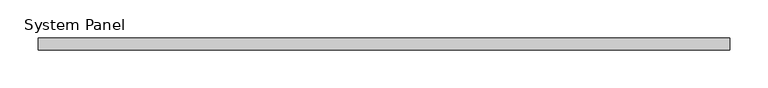
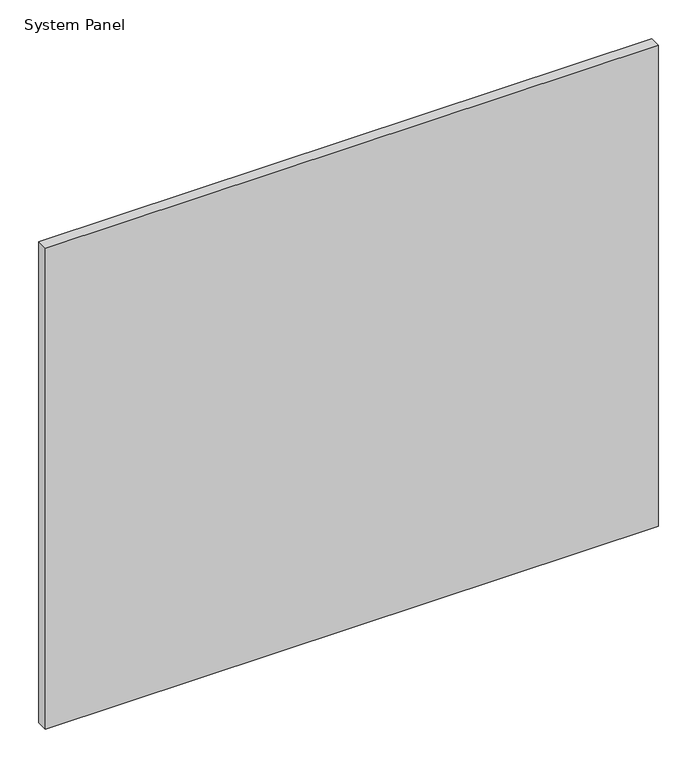
"""IFC4 building model written with IfcOpenShell, lengths in millimetres: plate geometry, System Panel : 로이복층유리_16."""

from ifc_helpers import new_model, si_unit, origin, origin_with_axes, place, context, project, spatial, polyline, outline, extrude, source, transform, mapped, element, save


def system_panel_34de0c9d(model_context):
    return source(origin(), model_context, "Body", "SweptSolid", [
        extrude(outline(polyline([(455.0, -8.0), (-455.0, -8.0), (-455.0, 8.0), (455.0, 8.0), (455.0, -8.0)])), origin_with_axes(), (0.0, 0.0, 1.0), 755.0),
    ])


if __name__ == "__main__":
    model = new_model("IFC4")
    model_context = context("Model", 3, world=origin())
    ifc_project = project(units=[si_unit("LENGTHUNIT", "METRE", prefix="MILLI")], contexts=[model_context])
    site = spatial("IfcSite", under=ifc_project)
    building = spatial("IfcBuilding", under=site)
    placement = place(None, origin())
    system_panel_shape = system_panel_34de0c9d(model_context)
    element("IfcPlate", 1, ObjectType="System Panel : 로이복층유리_16", at=placement, inside=building, context=model_context, shape_type="MappedRepresentation", body=[
        mapped(system_panel_shape, transform((0.0, 0.0, 0.0), x_axis=(1.0, 0.0, 0.0), y_axis=(0.0, 1.0, 0.0), z_axis=(0.0, 0.0, 1.0))),
    ])
    save(model, "model.ifc")

# Revit data of these elements
# Element 1 (IfcPlate, "System Panel : 로이복층유리_16")
#   Materials on its faces: "00_Glass_Glass"
# Materials
#   "00_Glass_Glass": class "Glass", colour RGB 218 227 224, transparency 0.85, Description = "Glass", Cost = 0, Image = none
